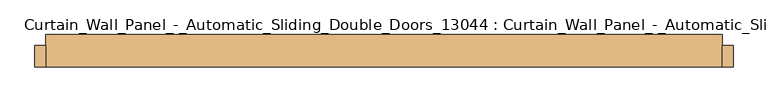
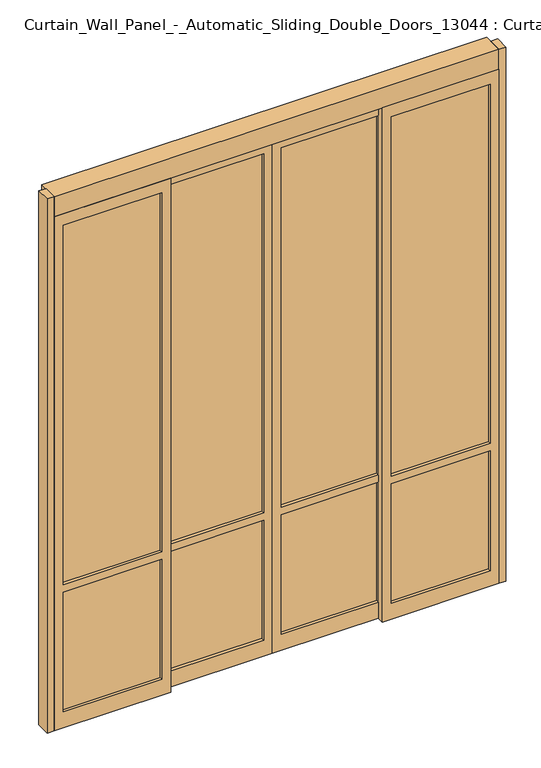
"""IFC4 building model written with IfcOpenShell, lengths in millimetres: door geometry, Curtain_Wall_Panel_-_Automatic_Sliding_Double_Doors_13044 : Curtain_Wall_Panel_-_Automatic_Sliding_Double_Doors_13044."""

from ifc_helpers import new_model, si_unit, frame, origin, origin_with_axes, place, context, project, spatial, polyline, outline, extrude, source, transform, mapped, element, save


def curtain_wall_panel_automatic_sliding_double_doors_13044_a9e0b89d(model_context):
    return source(origin(), model_context, "Body", "SweptSolid", [
        extrude(outline(polyline([(1536.7, -26.2355477), (1536.7, -35.3067868), (825.5, -35.3067868), (825.5, -26.2355477), (1536.7, -26.2355477)])), frame((0.0, 0.0, 120.65), z_axis=(0.0, 0.0, 1.0), x_axis=(1.0, 0.0, 0.0)), (0.0, 0.0, 1.0), 911.225),
        extrude(outline(polyline([(1536.7, -26.2355477), (1536.7, -35.3067868), (825.5, -35.3067868), (825.5, -26.2355477), (1536.7, -26.2355477)])), frame((0.0, 0.0, 1089.025), z_axis=(0.0, 0.0, 1.0), x_axis=(1.0, 0.0, 0.0)), (0.0, 0.0, 1.0), 2733.675),
        extrude(outline(polyline([(762.0, 25.6468909), (762.0, 16.0148002), (63.5, 16.0148002), (63.5, 25.6468909), (762.0, 25.6468909)])), frame((0.0, 0.0, 1089.025), z_axis=(0.0, 0.0, 1.0), x_axis=(1.0, 0.0, 0.0)), (0.0, 0.0, 1.0), 2733.675),
        extrude(outline(polyline([(762.0, 25.6468909), (762.0, 16.0148002), (63.5, 16.0148002), (63.5, 25.6468909), (762.0, 25.6468909)])), frame((0.0, 0.0, 120.65), z_axis=(0.0, 0.0, 1.0), x_axis=(1.0, 0.0, 0.0)), (0.0, 0.0, 1.0), 911.225),
        extrude(outline(polyline([(3911.6, 762.0), (0.0, 762.0), (0.0, 1600.2), (3911.6, 1600.2), (3911.6, 762.0)]), holes=[polyline([(1089.025, 825.5), (3822.7, 825.5), (3822.7, 1536.7), (1089.025, 1536.7), (1089.025, 825.5)]), polyline([(120.65, 1536.7), (120.65, 825.5), (1031.875, 825.5), (1031.875, 1536.7), (120.65, 1536.7)])]), frame((0.0, -57.15, 0.0), z_axis=(0.0, 1.0, 0.0), x_axis=(0.0, 0.0, 1.0)), (0.0, 0.0, 1.0), 50.8),
        extrude(outline(polyline([(3911.6, 825.5), (3911.6, 0.0), (0.0, 0.0), (0.0, 825.5), (3911.6, 825.5)]), holes=[polyline([(1031.875, 63.5), (1031.875, 762.0), (120.65, 762.0), (120.65, 63.5), (1031.875, 63.5)]), polyline([(3822.7, 762.0), (1089.025, 762.0), (1089.025, 63.5), (3822.7, 63.5), (3822.7, 762.0)])]), frame((0.0, -6.35, 0.0), z_axis=(0.0, 1.0, 0.0), x_axis=(0.0, 0.0, 1.0)), (0.0, 0.0, 1.0), 50.8),
        extrude(outline(polyline([(-825.5, -26.2355477), (-825.5, -35.3067868), (-1536.7, -35.3067868), (-1536.7, -26.2355477), (-825.5, -26.2355477)])), frame((0.0, 0.0, 1089.025), z_axis=(0.0, 0.0, 1.0), x_axis=(1.0, 0.0, 0.0)), (0.0, 0.0, 1.0), 2733.675),
        extrude(outline(polyline([(-825.5, -26.2355477), (-825.5, -35.3067868), (-1536.7, -35.3067868), (-1536.7, -26.2355477), (-825.5, -26.2355477)])), frame((0.0, 0.0, 120.65), z_axis=(0.0, 0.0, 1.0), x_axis=(1.0, 0.0, 0.0)), (0.0, 0.0, 1.0), 911.225),
        extrude(outline(polyline([(-63.5, 25.6468909), (-63.5, 16.0148002), (-762.0, 16.0148002), (-762.0, 25.6468909), (-63.5, 25.6468909)])), frame((0.0, 0.0, 120.65), z_axis=(0.0, 0.0, 1.0), x_axis=(1.0, 0.0, 0.0)), (0.0, 0.0, 1.0), 911.225),
        extrude(outline(polyline([(-63.5, 25.6468909), (-63.5, 16.0148002), (-762.0, 16.0148002), (-762.0, 25.6468909), (-63.5, 25.6468909)])), frame((0.0, 0.0, 1089.025), z_axis=(0.0, 0.0, 1.0), x_axis=(1.0, 0.0, 0.0)), (0.0, 0.0, 1.0), 2733.675),
        extrude(outline(polyline([(3911.6, -762.0), (3911.6, -1600.2), (0.0, -1600.2), (0.0, -762.0), (3911.6, -762.0)]), holes=[polyline([(1089.025, -825.5), (1089.025, -1536.7), (3822.7, -1536.7), (3822.7, -825.5), (1089.025, -825.5)]), polyline([(120.65, -1536.7), (1031.875, -1536.7), (1031.875, -825.5), (120.65, -825.5), (120.65, -1536.7)])]), frame((0.0, -57.15, 0.0), z_axis=(0.0, 1.0, 0.0), x_axis=(0.0, 0.0, 1.0)), (0.0, 0.0, 1.0), 50.8),
        extrude(outline(polyline([(3911.6, -825.5), (0.0, -825.5), (0.0, 0.0), (3911.6, 0.0), (3911.6, -825.5)]), holes=[polyline([(1031.875, -63.5), (120.65, -63.5), (120.65, -762.0), (1031.875, -762.0), (1031.875, -63.5)]), polyline([(3822.7, -762.0), (3822.7, -63.5), (1089.025, -63.5), (1089.025, -762.0), (3822.7, -762.0)])]), frame((0.0, -6.35, 0.0), z_axis=(0.0, 1.0, 0.0), x_axis=(0.0, 0.0, 1.0)), (0.0, 0.0, 1.0), 50.8),
        extrude(outline(polyline([(-1600.2, 44.45), (-1600.2, -57.15), (-1651.0, -57.15), (-1651.0, 44.45), (-1600.2, 44.45)])), origin_with_axes(), (0.0, 0.0, 1.0), 4064.0),
        extrude(outline(polyline([(1651.0, 44.45), (1651.0, -57.15), (1600.2, -57.15), (1600.2, 44.45), (1651.0, 44.45)])), origin_with_axes(), (0.0, 0.0, 1.0), 4064.0),
        extrude(outline(polyline([(1600.2, 95.25), (1600.2, -57.15), (-1600.2, -57.15), (-1600.2, 95.25), (1600.2, 95.25)])), frame((0.0, 0.0, 3911.6), z_axis=(0.0, 0.0, 1.0), x_axis=(1.0, 0.0, 0.0)), (0.0, 0.0, 1.0), 152.4),
    ])


if __name__ == "__main__":
    model = new_model("IFC4")
    model_context = context("Model", 3, world=origin())
    ifc_project = project(units=[si_unit("LENGTHUNIT", "METRE", prefix="MILLI")], contexts=[model_context])
    site = spatial("IfcSite", under=ifc_project)
    building = spatial("IfcBuilding", under=site)
    placement = place(None, origin())
    curtain_wall_panel_automatic_sliding_double_doors_13044_shape = curtain_wall_panel_automatic_sliding_double_doors_13044_a9e0b89d(model_context)
    element("IfcDoor", 1, ObjectType="Curtain_Wall_Panel_-_Automatic_Sliding_Double_Doors_13044 : Curtain_Wall_Panel_-_Automatic_Sliding_Double_Doors_13044", at=placement, inside=building, context=model_context, shape_type="MappedRepresentation", body=[
        mapped(curtain_wall_panel_automatic_sliding_double_doors_13044_shape, transform((0.0, 0.0, 0.0), x_axis=(1.0, 0.0, 0.0), y_axis=(0.0, 1.0, 0.0), z_axis=(0.0, 0.0, 1.0))),
    ])
    save(model, "model.ifc")

# Revit data of these elements
# Type "Curtain_Wall_Panel_-_Automatic_Sliding_Double_Doors_13044 : Curtain_Wall_Panel_-_Automatic_Sliding_Double_Doors_13044"
#   Type Mark = "22"
#   Frame Material = none
# Element 1 (IfcDoor, "Curtain_Wall_Panel_-_Automatic_Sliding_Double_Doors_13044 : Curtain_Wall_Panel_-_Automatic_Sliding_Double_Doors_13044")
#   Materials on its faces: "Glass"
# Materials
#   "Glass": class "Glass", colour RGB 0 128 192, transparency 0.75, Description = "Soda Lime Glass", Cost = 0
